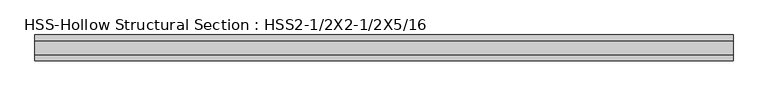
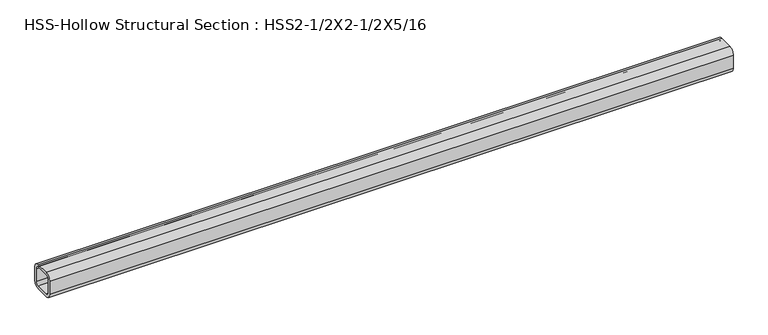
"""IFC4 building model written with IfcOpenShell, lengths in millimetres: beam geometry, HSS-Hollow Structural Section : HSS2-1/2X2-1/2X5/16."""

from ifc_helpers import new_model, si_unit, point, frame, frame_2d, origin, place, context, project, spatial, polyline, circle_curve, trimmed, segment, composite_curve, outline, extrude, source, transform, mapped, element, save


def hss_hollow_structural_section_hss2_1_2x2_1_2x5_16_3ef6e9af(model_context):
    return source(origin(), model_context, "Body", "SweptSolid", [
        extrude(outline(composite_curve([segment(polyline([(31.75, 16.9672), (31.75, -16.9672)]), True, "CONTINUOUS"), segment(trimmed(circle_curve(frame_2d((16.9672, -16.9672)), 14.7828), [point((31.75, -16.9672))], [point((16.9672, -31.75))], False, "CARTESIAN"), True, "CONTINUOUS"), segment(polyline([(16.9672, -31.75), (-16.9672, -31.75)]), True, "CONTINUOUS"), segment(trimmed(circle_curve(frame_2d((-16.9672, -16.9672)), 14.7828), [point((-16.9672, -31.75))], [point((-31.75, -16.9672))], False, "CARTESIAN"), True, "CONTINUOUS"), segment(polyline([(-31.75, -16.9672), (-31.75, 16.9672)]), True, "CONTINUOUS"), segment(trimmed(circle_curve(frame_2d((-16.9672, 16.9672)), 14.7828), [point((-31.75, 16.9672))], [point((-16.9672, 31.75))], False, "CARTESIAN"), True, "CONTINUOUS"), segment(polyline([(-16.9672, 31.75), (16.9672, 31.75)]), True, "CONTINUOUS"), segment(trimmed(circle_curve(frame_2d((16.9672, 16.9672)), 14.7828), [point((16.9672, 31.75))], [point((31.75, 16.9672))], False, "CARTESIAN"), True, "CONTINUOUS")], self_intersect=False), holes=[composite_curve([segment(trimmed(circle_curve(frame_2d((-16.9672, 16.9672)), 7.3914), [point((-16.9672, 24.3586))], [point((-24.3586, 16.9672))], True, "CARTESIAN"), True, "CONTINUOUS"), segment(polyline([(-24.3586, 16.9672), (-24.3586, -16.9672)]), True, "CONTINUOUS"), segment(trimmed(circle_curve(frame_2d((-16.9672, -16.9672)), 7.3914), [point((-24.3586, -16.9672))], [point((-16.9672, -24.3586))], True, "CARTESIAN"), True, "CONTINUOUS"), segment(polyline([(-16.9672, -24.3586), (16.9672, -24.3586)]), True, "CONTINUOUS"), segment(trimmed(circle_curve(frame_2d((16.9672, -16.9672)), 7.3914), [point((16.9672, -24.3586))], [point((24.3586, -16.9672))], True, "CARTESIAN"), True, "CONTINUOUS"), segment(polyline([(24.3586, -16.9672), (24.3586, 16.9672)]), True, "CONTINUOUS"), segment(trimmed(circle_curve(frame_2d((16.9672, 16.9672)), 7.3914), [point((24.3586, 16.9672))], [point((16.9672, 24.3586))], True, "CARTESIAN"), True, "CONTINUOUS"), segment(polyline([(16.9672, 24.3586), (-16.9672, 24.3586)]), True, "CONTINUOUS")], self_intersect=False)]), frame((-850.773, 0.0, 0.0), z_axis=(1.0, 0.0, 0.0), x_axis=(0.0, 1.0, 0.0)), (0.0, 0.0, 1.0), 1701.546),
    ])


if __name__ == "__main__":
    model = new_model("IFC4")
    model_context = context("Model", 3, world=origin())
    ifc_project = project(units=[si_unit("LENGTHUNIT", "METRE", prefix="MILLI")], contexts=[model_context])
    site = spatial("IfcSite", under=ifc_project)
    building = spatial("IfcBuilding", under=site)
    placement = place(None, origin())
    hss_hollow_structural_section_hss2_1_2x2_1_2x5_16_shape = hss_hollow_structural_section_hss2_1_2x2_1_2x5_16_3ef6e9af(model_context)
    element("IfcBeam", 1, ObjectType="HSS-Hollow Structural Section : HSS2-1/2X2-1/2X5/16", at=placement, inside=building, context=model_context, shape_type="MappedRepresentation", body=[
        mapped(hss_hollow_structural_section_hss2_1_2x2_1_2x5_16_shape, transform((0.0, 0.0, 0.0), x_axis=(1.0, 0.0, 0.0), y_axis=(0.0, 1.0, 0.0), z_axis=(0.0, 0.0, 1.0))),
    ])
    save(model, "model.ifc")

# Revit data of these elements
# Type "HSS-Hollow Structural Section : HSS2-1/2X2-1/2X5/16"
#   Assembly Code = "B10"
#   Shape = "Square"
#   W = 8.4
#   Ht = 0' - 2 1/2"
#   Length [instance default] = 5' - 0"
#   b = 0' - 2 1/2"
#   kr = 0' - 0.582"
#   t = 0' - 0.291"
#   A = 0.0163194 SF
#   Structural Material [instance default] = Steel ASTM A500, Grade B, Rectangular and Square
# Element 1 (IfcBeam, "HSS-Hollow Structural Section : HSS2-1/2X2-1/2X5/16")
#   Materials on its faces: "Steel ASTM A500, Grade B, Rectangular and Square"
# Materials
#   "Steel ASTM A500, Grade B, Rectangular and Square": class "Metal", colour RGB 199 199 199, transparency 0, Description = "Carbon steel", Cost = 0
